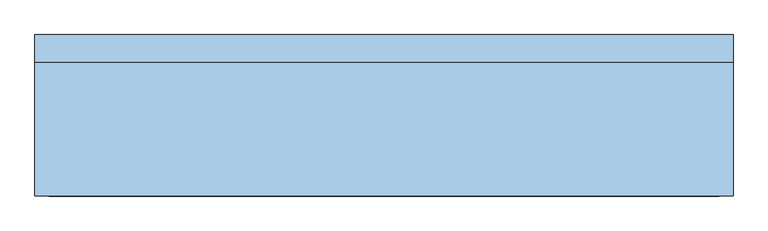
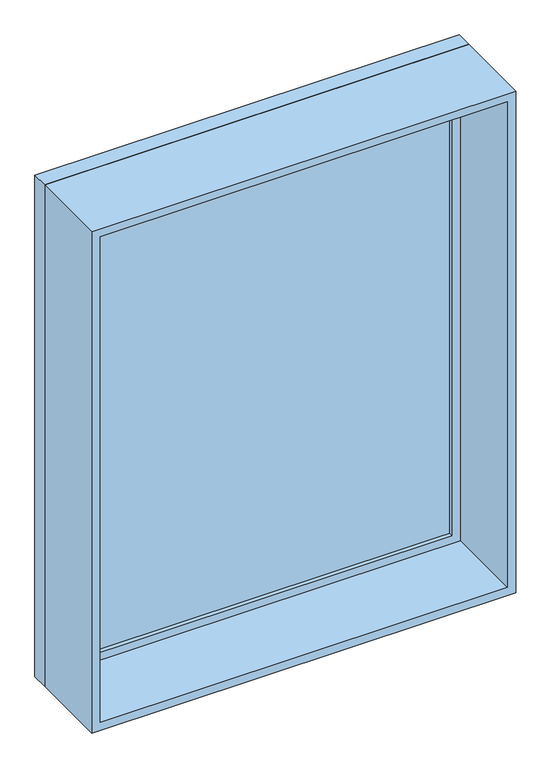
"""IFC4 building model written with IfcOpenShell, lengths in millimetres: window geometry, Фиксированные : 1600х2000."""

from ifc_helpers import new_model, si_unit, frame, origin, place, context, project, spatial, polyline, outline, extrude, source, transform, mapped, element, save


def window_c2055f4e(model_context):
    return source(origin(), model_context, "Body", "SweptSolid", [
        extrude(outline(polyline([(-737.0, 163.0), (737.0, 163.0), (737.0, 151.0), (-737.0, 151.0), (-737.0, 163.0)])), frame((0.0, 0.0, 978.0), z_axis=(0.0, 0.0, 1.0), x_axis=(1.0, 0.0, 0.0)), (0.0, 0.0, 1.0), 1874.0),
        extrude(outline(polyline([(2896.0, -781.0), (934.0, -781.0), (934.0, 781.0), (2896.0, 781.0), (2896.0, -781.0)]), holes=[polyline([(2852.0, -737.0), (2852.0, 737.0), (978.0, 737.0), (978.0, -737.0), (2852.0, -737.0)])]), frame((0.0, 135.0, 0.0), z_axis=(0.0, 1.0, 0.0), x_axis=(0.0, 0.0, 1.0)), (0.0, 0.0, 1.0), 44.0),
        extrude(outline(polyline([(2915.0, -800.0), (915.0, -800.0), (915.0, 800.0), (2915.0, 800.0), (2915.0, -800.0)]), holes=[polyline([(2896.0, -781.0), (2896.0, 781.0), (934.0, 781.0), (934.0, -781.0), (2896.0, -781.0)])]), frame((0.0, 135.0, 0.0), z_axis=(0.0, 1.0, 0.0), x_axis=(0.0, 0.0, 1.0)), (0.0, 0.0, 1.0), 63.0),
        extrude(outline(polyline([(2915.0, -800.0), (915.0, -800.0), (915.0, 800.0), (2915.0, 800.0), (2915.0, -800.0)]), holes=[polyline([(2883.0, -768.0), (2883.0, 768.0), (947.0, 768.0), (947.0, -768.0), (2883.0, -768.0)])]), frame((0.0, -172.0, 0.0), z_axis=(0.0, 1.0, 0.0), x_axis=(0.0, 0.0, 1.0)), (0.0, 0.0, 1.0), 307.0),
    ])


if __name__ == "__main__":
    model = new_model("IFC4")
    model_context = context("Model", 3, world=origin())
    ifc_project = project(units=[si_unit("LENGTHUNIT", "METRE", prefix="MILLI")], contexts=[model_context])
    site = spatial("IfcSite", under=ifc_project)
    building = spatial("IfcBuilding", under=site)
    placement = place(None, origin())
    window_shape = window_c2055f4e(model_context)
    element("IfcWindow", 1, ObjectType="Фиксированные : 1600х2000", at=placement, inside=building, context=model_context, shape_type="MappedRepresentation", body=[
        mapped(window_shape, transform((0.0, 0.0, 0.0), x_axis=(1.0, 0.0, 0.0), y_axis=(0.0, 1.0, 0.0), z_axis=(0.0, 0.0, 1.0))),
    ])
    save(model, "model.ifc")

# Revit data of these elements
# Type "Фиксированные : 1600х2000"
#   Type Mark = "20"
#   Construction Type Id = "GSP4R"
#   Analytic Construction = "Одинарное остекление стеклами Пилкингтон - 1/8 дюйма"
#   Visual Light Transmittance = 0.9
#   Solar Heat Gain Coefficient = 0.78
#   Heat Transfer Coefficient (U) = 3.6886 W/(m²·K)
#   Height = 2000 mm
#   Высота подоконника по умолчанию = 915 mm
#   Width = 1600 mm
#   Вставка окна = 19 mm
#   Наружный материал каркаса = Переплет
#   Внутренний материал каркаса = Переплет
#   Материал оконного стекла = Стекло
#   Переплет = Переплет
#   Wall Closure = (empty or 0)
# Element 1 (IfcWindow, "Фиксированные : 1600х2000")
#   Materials on its faces: "Переплет", "Стекло"
# Materials
#   "Переплет": class "Древесина", colour RGB 224 178 126, transparency 0, Cost = 0
#   "Стекло": class "Стекло", colour RGB 0 128 192, transparency 0.9, Description = "Известково-натриевое стекло", Cost = 0
